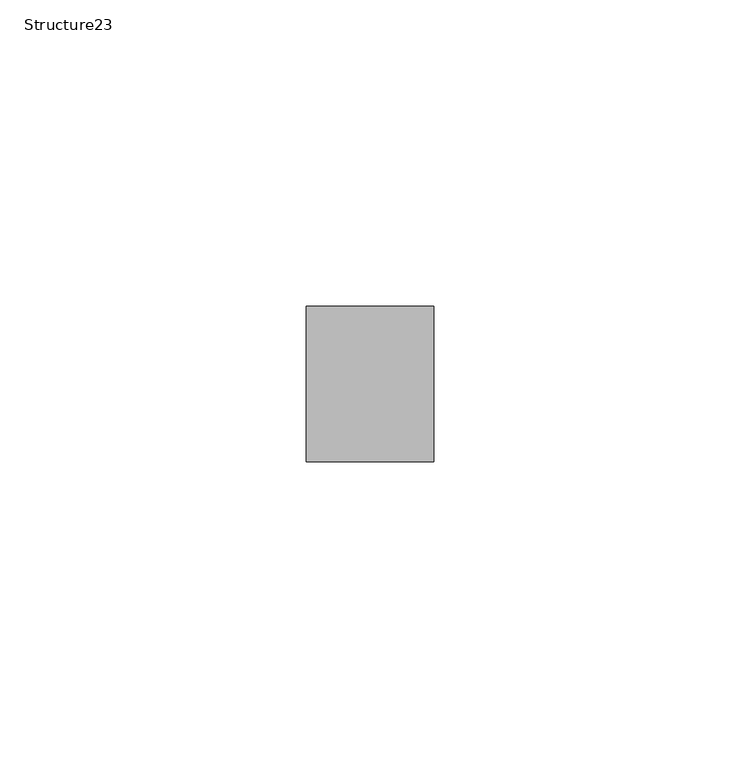
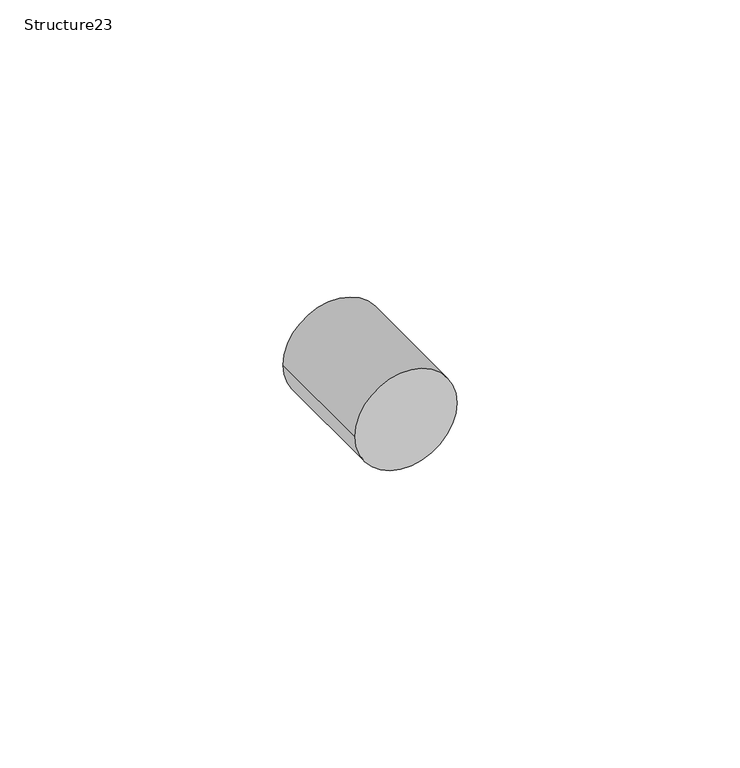
"""IFC4 building model written with IfcOpenShell, lengths in millimetres: proxy geometry, Structure23 : Structure668217151."""

from ifc_helpers import new_model, si_unit, point, frame, frame_2d, origin, place, context, project, spatial, circle_curve, trimmed, segment, composite_curve, outline, extrude, source, transform, mapped, element, save


def structure23_6975d512(model_context):
    return source(origin(), model_context, "Body", "SweptSolid", [
        extrude(outline(composite_curve([segment(trimmed(circle_curve(frame_2d((40908.7088339, 9847.8795269)), 10.4009751), [point((40908.7088339, 9837.4785517))], [point((40908.7088339, 9858.280502))], False, "CARTESIAN"), True, "CONTINUOUS"), segment(trimmed(circle_curve(frame_2d((40908.7088339, 9847.8795269)), 10.4009751), [point((40908.7088339, 9858.280502))], [point((40908.7088339, 9837.4785517))], False, "CARTESIAN"), True, "CONTINUOUS")], self_intersect=False)), frame((0.0, 1932.5073723, 0.0), z_axis=(0.0, 1.0, 0.0), x_axis=(0.0, 0.0, 1.0)), (0.0, 0.0, 1.0), 25.4),
    ])


if __name__ == "__main__":
    model = new_model("IFC4")
    model_context = context("Model", 3, world=origin())
    ifc_project = project(units=[si_unit("LENGTHUNIT", "METRE", prefix="MILLI")], contexts=[model_context])
    site = spatial("IfcSite", under=ifc_project)
    building = spatial("IfcBuilding", under=site)
    placement = place(None, origin())
    structure23_shape = structure23_6975d512(model_context)
    element("IfcBuildingElementProxy", 1, Name="Structure23 : Structure668217151", ObjectType="Structure23 : Structure668217151", at=placement, inside=building, context=model_context, shape_type="MappedRepresentation", body=[
        mapped(structure23_shape, transform((0.0, 0.0, 0.0), x_axis=(1.0, 0.0, 0.0), y_axis=(0.0, 1.0, 0.0), z_axis=(0.0, 0.0, 1.0))),
    ])
    save(model, "model.ifc")

# Revit data of these elements
# Type "Structure23 : Structure668217151"
#   NameOverride = "Structure668217151"
# Element 1 (IfcBuildingElementProxy, "Structure23 : Structure668217151")
#   Materials on its faces: "1.5\" DIA. STAINLESS STEEL RAILING"
# Materials
#   "1.5\" DIA. STAINLESS STEEL RAILING": class "Unassigned", colour RGB 128 128 128, transparency 0, Cost = 0
